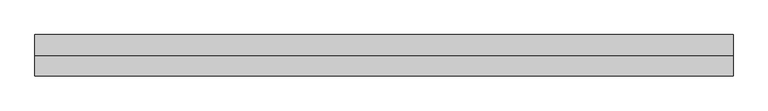
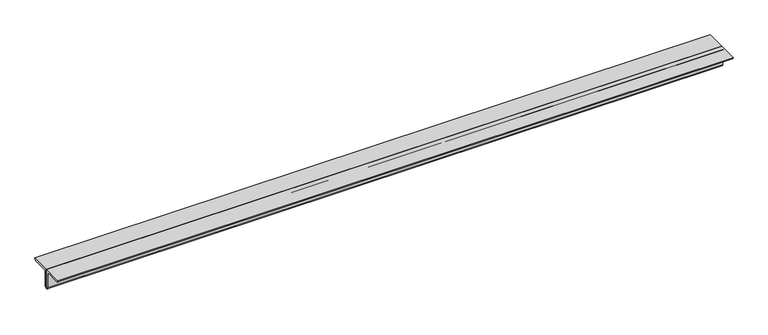
"""IFC4 building model written with IfcOpenShell, lengths in millimetres: member geometry, 0123_Steel Framing_2Ls-KSD3502 : H_SB_AR_S03_2Ls-130x130x12_HBR1."""

import ifcopenshell
import ifcopenshell.guid

model = None  # the IFC model being written
_history = None  # IfcOwnerHistory: only IFC2X3 demands one
_inside = {}  # id of a spatial element -> (the spatial element, [elements in it])
_under = {}  # id of a project, library or spatial element -> (it, [spatial elements below it])
_declared = {}  # id of a project -> (the project, [libraries it declares])
_typed = {}  # id of a type object -> (the type object, [elements of that type])
_made_of = {}  # id of a material, layer set ... -> (it, [elements and type objects made of it])


def new_model(schema):
    """Start an empty IFC model of exactly this schema.

    Asked for "IFC4X3", IfcOpenShell would pick the latest addendum, in which some entities
    have other attributes; the version numbers below select the first issue.
    IFC2X3 requires an IfcOwnerHistory on every rooted entity: one is made here for all.
    """
    global model, _history
    if schema == "IFC4X3":
        model = ifcopenshell.file(schema_version=(4, 3, 0, 0))
    else:
        model = ifcopenshell.file(schema=schema)
    _inside.clear()
    _under.clear()
    _declared.clear()
    _typed.clear()
    _made_of.clear()
    _history = None
    if model.schema == "IFC2X3":
        org = make("IfcOrganization", Name="unknown")
        user = make(
            "IfcPersonAndOrganization",
            ThePerson=make("IfcPerson", FamilyName="unknown"),
            TheOrganization=org,
        )
        app = make(
            "IfcApplication",
            ApplicationDeveloper=org,
            Version="unknown",
            ApplicationFullName="unknown",
            ApplicationIdentifier="unknown",
        )
        _history = make(
            "IfcOwnerHistory",
            OwningUser=user,
            OwningApplication=app,
            ChangeAction="ADDED",
            CreationDate=0,
        )
    return model


def make(cls, **values):
    """One entity of the class cls with the attributes given. An attribute that is None is left unset."""
    return model.create_entity(
        cls, **{name: value for name, value in values.items() if value is not None}
    )


def rooted(cls, **values):
    """An entity with a GlobalId (a new one), such as an element, a storey or a relation."""
    return make(cls, GlobalId=ifcopenshell.guid.new(), OwnerHistory=_history, **values)


def si_unit(unit_type, name, prefix=None):
    """IfcSIUnit, for example si_unit("LENGTHUNIT", "METRE", prefix="MILLI")."""
    return make("IfcSIUnit", UnitType=unit_type, Prefix=prefix, Name=name)


def assignment(units):
    """IfcUnitAssignment: the units of a project."""
    return None if units is None else make("IfcUnitAssignment", Units=units)


def point(xyz):
    """IfcCartesianPoint."""
    return None if xyz is None else make("IfcCartesianPoint", Coordinates=xyz)


def direction(xyz):
    """IfcDirection."""
    return None if xyz is None else make("IfcDirection", DirectionRatios=xyz)


def frame(location, z_axis=None, x_axis=None):
    """IfcAxis2Placement3D, a coordinate frame: its origin and axes. An axis left out is left unset."""
    return make(
        "IfcAxis2Placement3D",
        Location=point(location),
        Axis=direction(z_axis),
        RefDirection=direction(x_axis),
    )


def frame_2d(location, x_axis=None):
    """IfcAxis2Placement2D, a coordinate frame in the plane: its origin and x axis."""
    return make(
        "IfcAxis2Placement2D", Location=point(location), RefDirection=direction(x_axis)
    )


def origin():
    """The frame at (0, 0, 0) with its axes left unset."""
    return frame((0.0, 0.0, 0.0))


def place(relative_to, where):
    """IfcLocalPlacement: puts the frame where relative to a parent placement (None: the world)."""
    return make(
        "IfcLocalPlacement", PlacementRelTo=relative_to, RelativePlacement=where
    )


def context(
    kind, dimensions, precision=None, world=None, true_north=None, identifier=None
):
    """IfcGeometricRepresentationContext, for example the 3D "Model" context."""
    return make(
        "IfcGeometricRepresentationContext",
        ContextIdentifier=identifier,
        ContextType=kind,
        CoordinateSpaceDimension=dimensions,
        Precision=precision,
        WorldCoordinateSystem=world,
        TrueNorth=true_north,
    )


def project(units=None, contexts=None):
    """IfcProject with its units and contexts."""
    return rooted(
        "IfcProject",
        Name="project",
        RepresentationContexts=contexts,
        UnitsInContext=assignment(units),
    )


def spatial(cls, under=None, at=None, **own):
    """A site, building, storey or space (cls), placed at a placement, below another one or the project."""
    s = rooted(cls, ObjectPlacement=at, **own)
    if under is not None:
        _under.setdefault(under.id(), (under, []))[1].append(s)
    return s


def polyline(points):
    """IfcPolyline through the points."""
    return make("IfcPolyline", Points=[point(p) for p in points])


def circle_curve(where, radius):
    """IfcCircle in the frame where."""
    return make("IfcCircle", Position=where, Radius=radius)


def trimmed(basis, trim1, trim2, sense, master):
    """IfcTrimmedCurve: the piece of a basis curve between two trims."""
    return make(
        "IfcTrimmedCurve",
        BasisCurve=basis,
        Trim1=trim1,
        Trim2=trim2,
        SenseAgreement=sense,
        MasterRepresentation=master,
    )


def segment(curve, same_sense, transition):
    """IfcCompositeCurveSegment."""
    return make(
        "IfcCompositeCurveSegment",
        Transition=transition,
        SameSense=same_sense,
        ParentCurve=curve,
    )


def composite_curve(segments, self_intersect=None):
    """IfcCompositeCurve: segments joined end to end."""
    return make("IfcCompositeCurve", Segments=segments, SelfIntersect=self_intersect)


def outline(outer, holes=None, kind="AREA"):
    """IfcArbitraryClosedProfileDef: a profile drawn as a closed curve; with holes, ...WithVoids."""
    if holes is None:
        return make("IfcArbitraryClosedProfileDef", ProfileType=kind, OuterCurve=outer)
    return make(
        "IfcArbitraryProfileDefWithVoids",
        ProfileType=kind,
        OuterCurve=outer,
        InnerCurves=holes,
    )


def extrude(swept, where, along, depth):
    """IfcExtrudedAreaSolid: the profile swept, set in the frame where, extruded along a direction by depth."""
    return make(
        "IfcExtrudedAreaSolid",
        SweptArea=swept,
        Position=where,
        ExtrudedDirection=direction(along),
        Depth=depth,
    )


def shape(context_of_items, identifier, shape_type, items):
    """IfcShapeRepresentation: the items that make up one representation, for example the "Body"."""
    return make(
        "IfcShapeRepresentation",
        ContextOfItems=context_of_items,
        RepresentationIdentifier=identifier,
        RepresentationType=shape_type,
        Items=items,
    )


def source(mapping_origin, context_of_items, identifier, shape_type, items):
    """IfcRepresentationMap: a shape defined once, which mapped items show again and again."""
    return make(
        "IfcRepresentationMap",
        MappingOrigin=mapping_origin,
        MappedRepresentation=shape(context_of_items, identifier, shape_type, items),
    )


def transform(
    local_origin,
    x_axis=None,
    y_axis=None,
    z_axis=None,
    scale=None,
    scale2=None,
    scale3=None,
    uniform=True,
):
    """IfcCartesianTransformationOperator3D, or its non-uniform kind. x_axis, y_axis, z_axis: its Axis1, 2, 3."""
    if uniform:
        return make(
            "IfcCartesianTransformationOperator3D",
            Axis1=direction(x_axis),
            Axis2=direction(y_axis),
            LocalOrigin=point(local_origin),
            Scale=scale,
            Axis3=direction(z_axis),
        )
    return make(
        "IfcCartesianTransformationOperator3DnonUniform",
        Axis1=direction(x_axis),
        Axis2=direction(y_axis),
        LocalOrigin=point(local_origin),
        Scale=scale,
        Axis3=direction(z_axis),
        Scale2=scale2,
        Scale3=scale3,
    )


def mapped(mapping_source, mapping_target):
    """IfcMappedItem: shows the shape of a source again, moved by a transform."""
    return make(
        "IfcMappedItem", MappingSource=mapping_source, MappingTarget=mapping_target
    )


def made_of(thing, what):
    """Note that an element or type object is made of a material, layer set ...; save() writes the relation."""
    if what is not None:
        _made_of.setdefault(what.id(), (what, []))[1].append(thing)
    return thing


def element(
    cls,
    number,
    at=None,
    inside=None,
    cuts=None,
    type_object=None,
    material=None,
    context=None,
    identifier="Body",
    shape_type=None,
    held_by="IfcProductDefinitionShape",
    body=None,
    shapes=None,
    **own,
):
    """One element of the class cls, such as IfcWall. Its Tag is "e" and its number.

    at: its placement. inside: the storey or other place that contains it. cuts: it is an
    opening in that element (IfcRelVoidsElement). A single representation is given by context,
    identifier, shape_type and body (its items); several are given by shapes. held_by: the class
    of the entity that holds the representations. save() writes the other relations.
    """
    e = rooted(cls, Tag="e%d" % number, ObjectPlacement=at, **own)
    if body is not None:
        shapes = [shape(context, identifier, shape_type, body)]
    if shapes is not None:
        e.Representation = make(held_by, Representations=shapes)
    if inside is not None:
        _inside.setdefault(inside.id(), (inside, []))[1].append(e)
    if cuts is not None:
        rooted(
            "IfcRelVoidsElement", RelatingBuildingElement=cuts, RelatedOpeningElement=e
        )
    if type_object is not None:
        _typed.setdefault(type_object.id(), (type_object, []))[1].append(e)
    return made_of(e, material)


def aggregate(whole, parts):
    """IfcRelAggregates: a whole, such as a stair, and the parts it consists of."""
    return rooted("IfcRelAggregates", RelatingObject=whole, RelatedObjects=parts)


def save(model, path):
    """Write the relations noted so far, then the file.

    IfcRelAggregates (storeys below a building ...), IfcRelContainedInSpatialStructure (elements
    in a storey), IfcRelDefinesByType, IfcRelAssociatesMaterial and IfcRelDeclares: one each for
    every whole, place, type object, material and project.
    """
    for whole, parts in _under.values():
        aggregate(whole, parts)
    for where, things in _inside.values():
        rooted(
            "IfcRelContainedInSpatialStructure",
            RelatedElements=things,
            RelatingStructure=where,
        )
    for kind, things in _typed.values():
        rooted("IfcRelDefinesByType", RelatedObjects=things, RelatingType=kind)
    for what, things in _made_of.values():
        rooted("IfcRelAssociatesMaterial", RelatedObjects=things, RelatingMaterial=what)
    for by, libraries in _declared.values():
        rooted("IfcRelDeclares", RelatingContext=by, RelatedDefinitions=libraries)
    model.write(path)


def member_50d2e036(model_context):
    return source(origin(), model_context, "Body", "SweptSolid", [
        extrude(outline(composite_curve([segment(polyline([(0.0, 36.4), (130.0, 36.4)]), True, "CONTINUOUS"), segment(trimmed(circle_curve(frame_2d((118.0, 36.4)), 12.0), [point((130.0, 36.4))], [point((118.0, 24.4))], False, "CARTESIAN"), True, "CONTINUOUS"), segment(polyline([(118.0, 24.4), (24.0, 24.4)]), True, "CONTINUOUS"), segment(trimmed(circle_curve(frame_2d((24.0, 12.4)), 12.0), [point((24.0, 24.4))], [point((12.0, 12.4))], True, "CARTESIAN"), True, "CONTINUOUS"), segment(polyline([(12.0, 12.4), (12.0, -81.6)]), True, "CONTINUOUS"), segment(trimmed(circle_curve(frame_2d((0.0, -81.6)), 12.0), [point((12.0, -81.6))], [point((0.0, -93.6))], False, "CARTESIAN"), True, "CONTINUOUS"), segment(polyline([(0.0, -93.6), (0.0, 36.4)]), True, "CONTINUOUS")], self_intersect=False)), frame((-2203.0201459, 0.0, 0.0), z_axis=(1.0, 0.0, 0.0), x_axis=(0.0, 1.0, 0.0)), (0.0, 0.0, 1.0), 4391.0649986),
        extrude(outline(composite_curve([segment(polyline([(0.0, 36.4), (0.0, -93.6)]), True, "CONTINUOUS"), segment(trimmed(circle_curve(frame_2d((0.0, -81.6)), 12.0), [point((0.0, -93.6))], [point((-12.0, -81.6))], False, "CARTESIAN"), True, "CONTINUOUS"), segment(polyline([(-12.0, -81.6), (-12.0, 12.4)]), True, "CONTINUOUS"), segment(trimmed(circle_curve(frame_2d((-24.0, 12.4)), 12.0), [point((-12.0, 12.4))], [point((-24.0, 24.4))], True, "CARTESIAN"), True, "CONTINUOUS"), segment(polyline([(-24.0, 24.4), (-118.0, 24.4)]), True, "CONTINUOUS"), segment(trimmed(circle_curve(frame_2d((-118.0, 36.4)), 12.0), [point((-118.0, 24.4))], [point((-130.0, 36.4))], False, "CARTESIAN"), True, "CONTINUOUS"), segment(polyline([(-130.0, 36.4), (0.0, 36.4)]), True, "CONTINUOUS")], self_intersect=False)), frame((-2203.0201459, 0.0, 0.0), z_axis=(1.0, 0.0, 0.0), x_axis=(0.0, 1.0, 0.0)), (0.0, 0.0, 1.0), 4391.0649986),
    ])


if __name__ == "__main__":
    model = new_model("IFC4")
    model_context = context("Model", 3, world=origin())
    ifc_project = project(units=[si_unit("LENGTHUNIT", "METRE", prefix="MILLI")], contexts=[model_context])
    site = spatial("IfcSite", under=ifc_project)
    building = spatial("IfcBuilding", under=site)
    placement = place(None, origin())
    member_shape = member_50d2e036(model_context)
    element("IfcMember", 1, ObjectType="0123_Steel Framing_2Ls-KSD3502 : H_SB_AR_S03_2Ls-130x130x12_HBR1", at=placement, inside=building, context=model_context, shape_type="MappedRepresentation", body=[
        mapped(member_shape, transform((0.0, 0.0, 0.0), x_axis=(1.0, 0.0, 0.0), y_axis=(0.0, 1.0, 0.0), z_axis=(0.0, 0.0, 1.0))),
    ])
    save(model, "model.ifc")

# Revit data of these elements
# Type "0123_Steel Framing_2Ls-KSD3502 : H_SB_AR_S03_2Ls-130x130x12_HBR1"
#   Type Mark = "HBR1"
#   Assembly Code = "B10"
#   Legs = "SLBB"
#   W = 8.97
#   Perimeter = 1.04 m²/m
#   Nominal Weight = 46.80 kgf/m
#   Length [instance default] = 1000 mm
#   Space = 0 mm
#   b = 130 mm
#   d = 130 mm
#   t = 12 mm
#   y = 36.4 mm
#   A = 0.005952 m²
#   Structural Material [instance default] = Steel ASTM A36
# Element 1 (IfcMember, "0123_Steel Framing_2Ls-KSD3502 : H_SB_AR_S03_2Ls-130x130x12_HBR1")
#   Materials on its faces: "Steel ASTM A36"
# Materials
#   "Steel ASTM A36": class "Metal", colour RGB 199 199 199, transparency 0, Description = "Structural steel, ASTM A36 Grade B, mill finish", Cost = 0
